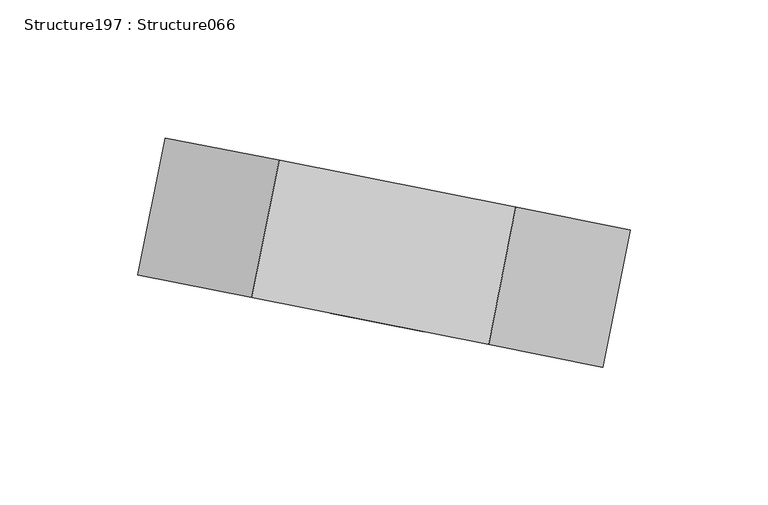
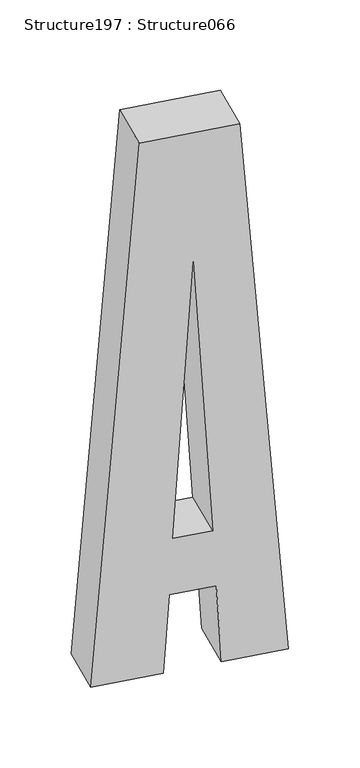
"""IFC4 building model written with IfcOpenShell, lengths in millimetres: proxy geometry, Structure197 : Structure066."""

from ifc_helpers import new_model, si_unit, frame, origin, place, context, project, spatial, polyline, outline, extrude, source, transform, mapped, element, save


def structure197_structure066_595a767e(model_context):
    return source(origin(), model_context, "Body", "SweptSolid", [
        extrude(outline(polyline([(58.3911478, 0.0), (16.1366011, -537.7810299), (-71.4467402, -537.7810299), (-113.6959495, 0.0), (-50.7062387, 0.0), (-45.322746, -77.5877646), (-4.6017654, -77.5877646), (0.0, 0.0), (58.3911478, 0.0)]), holes=[polyline([(-7.6792161, -133.6760727), (-42.2492093, -133.6760727), (-24.5840236, -407.952749), (-7.6792161, -133.6760727)])]), frame((-1941.72426, 234853.829899, 595.2038833), z_axis=(0.1946622229639412, 0.9808703374813293, 0.0), x_axis=(0.9808703374813293, -0.1946622229639412, 0.0)), (0.0, 0.0, 1.0), 50.8),
    ])


if __name__ == "__main__":
    model = new_model("IFC4")
    model_context = context("Model", 3, world=origin())
    ifc_project = project(units=[si_unit("LENGTHUNIT", "METRE", prefix="MILLI")], contexts=[model_context])
    site = spatial("IfcSite", under=ifc_project)
    building = spatial("IfcBuilding", under=site)
    placement = place(None, origin())
    structure197_structure066_shape = structure197_structure066_595a767e(model_context)
    element("IfcBuildingElementProxy", 1, Name="Structure197 : Structure066", ObjectType="Structure197 : Structure066", at=placement, inside=building, context=model_context, shape_type="MappedRepresentation", body=[
        mapped(structure197_structure066_shape, transform((0.0, 0.0, 0.0), x_axis=(1.0, 0.0, 0.0), y_axis=(0.0, 1.0, 0.0), z_axis=(0.0, 0.0, 1.0))),
    ])
    save(model, "model.ifc")

# Revit data of these elements
# Type "Structure197 : Structure066"
#   NameOverride = "Structure066"
# Element 1 (IfcBuildingElementProxy, "Structure197 : Structure066")
#   Materials on its faces: "BRUSHED ALUMINUM LETTERING"
# Materials
#   "BRUSHED ALUMINUM LETTERING": class "Unassigned", colour RGB 169 181 186, transparency 0, Cost = 0
